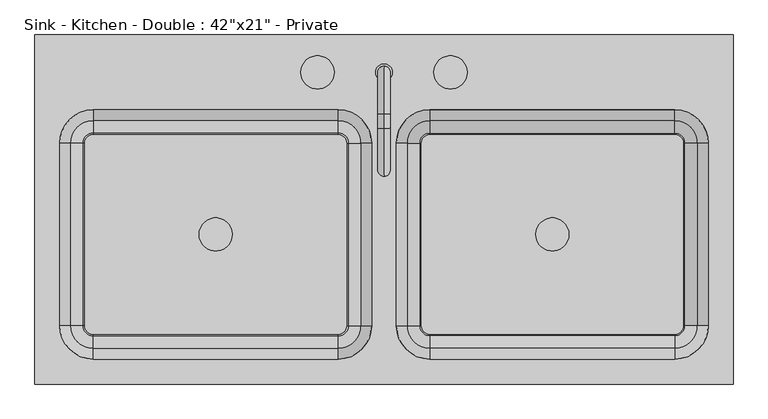
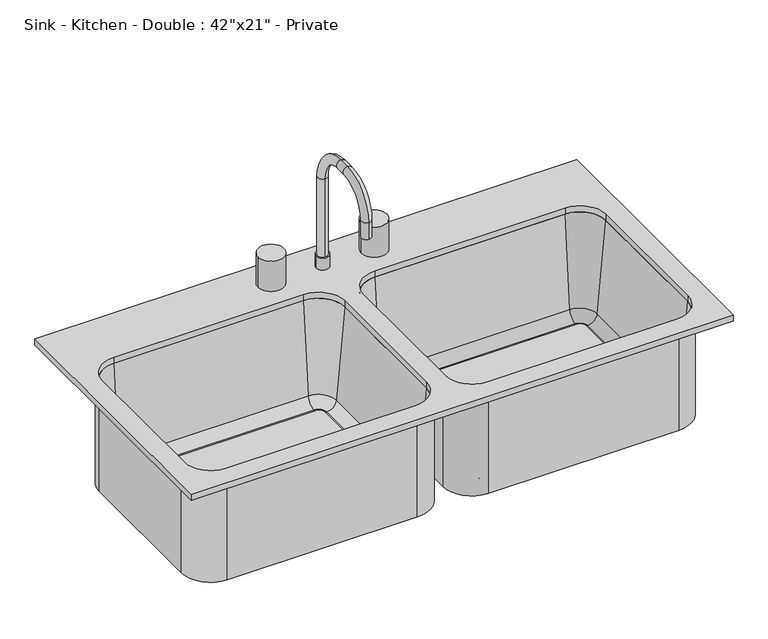
"""IFC4 building model written with IfcOpenShell, lengths in millimetres: flow terminal geometry."""

from ifc_helpers import new_model, si_unit, point, frame, frame_2d, origin, origin_with_axes, place, context, project, spatial, polyline, circle_curve, ellipse_curve, trimmed, segment, composite_curve, outline, extrude, source, transform, mapped, element, save
from ifc_brep_helpers import plane_surface, cylinder_surface, revolved_surface, advanced_brep


def flow_terminal_ad7a5719(model_context):
    return source(origin(), model_context, "Body", "SolidModel", [
        extrude(outline(composite_curve([segment(trimmed(circle_curve(frame_2d((444.5, -165.1)), 12.7), [point((444.5, -152.4))], [point((457.2, -165.1))], False, "CARTESIAN"), True, "CONTINUOUS"), segment(polyline([(457.2, -165.1), (457.2, -444.5)]), True, "CONTINUOUS"), segment(trimmed(circle_curve(frame_2d((444.5, -444.5)), 12.7), [point((457.2, -444.5))], [point((444.5, -457.2))], False, "CARTESIAN"), True, "CONTINUOUS"), segment(polyline([(444.5, -457.2), (69.85, -457.2)]), True, "CONTINUOUS"), segment(trimmed(circle_curve(frame_2d((69.85, -444.5)), 12.7), [point((69.85, -457.2))], [point((57.15, -444.5))], False, "CARTESIAN"), True, "CONTINUOUS"), segment(polyline([(57.15, -444.5), (57.15, -165.1)]), True, "CONTINUOUS"), segment(trimmed(circle_curve(frame_2d((69.85, -165.1)), 12.7), [point((57.15, -165.1))], [point((69.85, -152.4))], False, "CARTESIAN"), True, "CONTINUOUS"), segment(polyline([(69.85, -152.4), (444.5, -152.4)]), True, "CONTINUOUS")], self_intersect=False), holes=[composite_curve([segment(trimmed(circle_curve(frame_2d((257.175, -304.8)), 25.4), [point((231.775, -304.8))], [point((282.575, -304.8))], True, "CARTESIAN"), True, "CONTINUOUS"), segment(trimmed(circle_curve(frame_2d((257.175, -304.8)), 25.4), [point((282.575, -304.8))], [point((231.775, -304.8))], True, "CARTESIAN"), True, "CONTINUOUS")], self_intersect=False)]), frame((0.0, 0.0, -215.9), z_axis=(0.0, 0.0, 1.0), x_axis=(1.0, 0.0, 0.0)), (0.0, 0.0, 1.0), 9.525),
        advanced_brep(
        [(19.05, -165.1, 0.0), (69.85, -114.3, 0.0), (69.85, -107.95, 0.0), (12.7, -165.1, 0.0), (35.5840728, -165.1, -188.9853169), (69.85, -130.8340728, -188.9853169), (54.5615818, -165.1, -206.375), (69.85, -149.8115818, -206.375), (57.15, -165.1, -206.375), (69.85, -152.4, -206.375), (57.15, -165.1, -215.9), (69.85, -152.4, -215.9), (12.7, -165.1, -215.9), (69.85, -107.95, -215.9), (12.7, -444.5, 0.0), (19.05, -444.5, 0.0), (35.5840728, -444.5, -188.9853169), (54.5615818, -444.5, -206.375), (57.15, -444.5, -206.375), (57.15, -444.5, -215.9), (12.7, -444.5, -215.9), (69.85, -495.3, 0.0), (69.85, -501.65, 0.0), (69.85, -478.7659272, -188.9853169), (69.85, -459.7884182, -206.375), (69.85, -457.2, -206.375), (69.85, -457.2, -215.9), (69.85, -501.65, -215.9), (444.5, -501.65, 0.0), (444.5, -495.3, 0.0), (444.5, -478.7659272, -188.9853169), (444.5, -459.7884182, -206.375), (444.5, -457.2, -206.375), (444.5, -457.2, -215.9), (444.5, -501.65, -215.9), (495.3, -444.5, 0.0), (501.65, -444.5, 0.0), (478.7659272, -444.5, -188.9853169), (459.7884182, -444.5, -206.375), (457.2, -444.5, -206.375), (457.2, -444.5, -215.9), (501.65, -444.5, -215.9), (501.65, -165.1, 0.0), (495.3, -165.1, 0.0), (478.7659272, -165.1, -188.9853169), (459.7884182, -165.1, -206.375), (457.2, -165.1, -206.375), (457.2, -165.1, -215.9), (501.65, -165.1, -215.9), (444.5, -114.3, 0.0), (444.5, -107.95, 0.0), (444.5, -130.8340728, -188.9853169), (444.5, -149.8115818, -206.375), (444.5, -152.4, -206.375), (444.5, -152.4, -215.9), (444.5, -107.95, -215.9)],
        [
            (0, 1, circle_curve(frame((69.85, -165.1, 0.0), z_axis=(0.0, 0.0, -1.0), x_axis=(0.0, 1.0, 0.0)), 50.8)),
            (1, 2),
            (2, 3, circle_curve(frame((69.85, -165.1, 0.0), z_axis=(0.0, 0.0, 1.0), x_axis=(0.0, 1.0, 0.0)), 57.15)),
            (3, 0),
            (4, 5, circle_curve(frame((69.85, -165.1, -188.9853169), z_axis=(0.0, 0.0, -1.0), x_axis=(0.0, 1.0, 0.0)), 34.2659272)),
            (5, 1),
            (0, 4),
            (6, 7, circle_curve(frame((69.85, -165.1, -206.375), z_axis=(0.0, 0.0, -1.0), x_axis=(0.0, 1.0, 0.0)), 15.2884182)),
            (7, 5, circle_curve(frame((69.85, -149.8115818, -187.325), z_axis=(1.0, 0.0, 0.0), x_axis=(0.0, -1.0, 0.0)), 19.05)),
            (4, 6, circle_curve(frame((54.5615818, -165.1, -187.325), z_axis=(0.0, -1.0, 0.0), x_axis=(1.0, 0.0, 0.0)), 19.05)),
            (8, 9, circle_curve(frame((69.85, -165.1, -206.375), z_axis=(0.0, 0.0, -1.0), x_axis=(0.0, 1.0, 0.0)), 12.7)),
            (9, 7),
            (6, 8),
            (10, 11, circle_curve(frame((69.85, -165.1, -215.9), z_axis=(0.0, 0.0, -1.0), x_axis=(0.0, 1.0, 0.0)), 12.7)),
            (11, 9),
            (8, 10),
            (12, 13, circle_curve(frame((69.85, -165.1, -215.9), z_axis=(0.0, 0.0, -1.0), x_axis=(0.0, 1.0, 0.0)), 57.15)),
            (13, 11),
            (10, 12),
            (2, 13),
            (12, 3),
            (3, 14),
            (14, 15),
            (15, 0),
            (15, 16),
            (16, 4),
            (16, 17, circle_curve(frame((54.5615818, -444.5, -187.325), z_axis=(0.0, -1.0, 0.0), x_axis=(1.0, 0.0, 0.0)), 19.05)),
            (17, 6),
            (17, 18),
            (18, 8),
            (18, 19),
            (19, 10),
            (19, 20),
            (20, 12),
            (20, 14),
            (21, 15, circle_curve(frame((69.85, -444.5, 0.0), z_axis=(0.0, 0.0, -1.0), x_axis=(-1.0, 0.0, 0.0)), 50.8)),
            (14, 22, circle_curve(frame((69.85, -444.5, 0.0), z_axis=(0.0, 0.0, 1.0), x_axis=(-1.0, 0.0, 0.0)), 57.15)),
            (22, 21),
            (23, 16, circle_curve(frame((69.85, -444.5, -188.9853169), z_axis=(0.0, 0.0, -1.0), x_axis=(-1.0, 0.0, 0.0)), 34.2659272)),
            (21, 23),
            (24, 17, circle_curve(frame((69.85, -444.5, -206.375), z_axis=(0.0, 0.0, -1.0), x_axis=(-1.0, 0.0, 0.0)), 15.2884182)),
            (23, 24, circle_curve(frame((69.85, -459.7884182, -187.325), z_axis=(1.0, 0.0, 0.0), x_axis=(0.0, 1.0, 0.0)), 19.05)),
            (25, 18, circle_curve(frame((69.85, -444.5, -206.375), z_axis=(0.0, 0.0, -1.0), x_axis=(-1.0, 0.0, 0.0)), 12.7)),
            (24, 25),
            (26, 19, circle_curve(frame((69.85, -444.5, -215.9), z_axis=(0.0, 0.0, -1.0), x_axis=(-1.0, 0.0, 0.0)), 12.7)),
            (25, 26),
            (27, 20, circle_curve(frame((69.85, -444.5, -215.9), z_axis=(0.0, 0.0, -1.0), x_axis=(-1.0, 0.0, 0.0)), 57.15)),
            (26, 27),
            (27, 22),
            (22, 28),
            (28, 29),
            (29, 21),
            (29, 30),
            (30, 23),
            (30, 31, circle_curve(frame((444.5, -459.7884182, -187.325), z_axis=(1.0, 0.0, 0.0), x_axis=(0.0, 1.0, 0.0)), 19.05)),
            (31, 24),
            (31, 32),
            (32, 25),
            (32, 33),
            (33, 26),
            (33, 34),
            (34, 27),
            (34, 28),
            (35, 29, circle_curve(frame((444.5, -444.5, 0.0), z_axis=(0.0, 0.0, -1.0), x_axis=(0.0, -1.0, 0.0)), 50.8)),
            (28, 36, circle_curve(frame((444.5, -444.5, 0.0), z_axis=(0.0, 0.0, 1.0), x_axis=(0.0, -1.0, 0.0)), 57.15)),
            (36, 35),
            (37, 30, circle_curve(frame((444.5, -444.5, -188.9853169), z_axis=(0.0, 0.0, -1.0), x_axis=(0.0, -1.0, 0.0)), 34.2659272)),
            (35, 37),
            (38, 31, circle_curve(frame((444.5, -444.5, -206.375), z_axis=(0.0, 0.0, -1.0), x_axis=(0.0, -1.0, 0.0)), 15.2884182)),
            (37, 38, circle_curve(frame((459.7884182, -444.5, -187.325), z_axis=(0.0, 1.0, 0.0), x_axis=(-1.0, 0.0, 0.0)), 19.05)),
            (39, 32, circle_curve(frame((444.5, -444.5, -206.375), z_axis=(0.0, 0.0, -1.0), x_axis=(0.0, -1.0, 0.0)), 12.7)),
            (38, 39),
            (40, 33, circle_curve(frame((444.5, -444.5, -215.9), z_axis=(0.0, 0.0, -1.0), x_axis=(0.0, -1.0, 0.0)), 12.7)),
            (39, 40),
            (41, 34, circle_curve(frame((444.5, -444.5, -215.9), z_axis=(0.0, 0.0, -1.0), x_axis=(0.0, -1.0, 0.0)), 57.15)),
            (40, 41),
            (41, 36),
            (36, 42),
            (42, 43),
            (43, 35),
            (43, 44),
            (44, 37),
            (44, 45, circle_curve(frame((459.7884182, -165.1, -187.325), z_axis=(0.0, 1.0, 0.0), x_axis=(-1.0, 0.0, 0.0)), 19.05)),
            (45, 38),
            (45, 46),
            (46, 39),
            (46, 47),
            (47, 40),
            (47, 48),
            (48, 41),
            (48, 42),
            (49, 43, circle_curve(frame((444.5, -165.1, 0.0), z_axis=(0.0, 0.0, -1.0), x_axis=(1.0, 0.0, 0.0)), 50.8)),
            (42, 50, circle_curve(frame((444.5, -165.1, 0.0), z_axis=(0.0, 0.0, 1.0), x_axis=(1.0, 0.0, 0.0)), 57.15)),
            (50, 49),
            (51, 44, circle_curve(frame((444.5, -165.1, -188.9853169), z_axis=(0.0, 0.0, -1.0), x_axis=(1.0, 0.0, 0.0)), 34.2659272)),
            (49, 51),
            (52, 45, circle_curve(frame((444.5, -165.1, -206.375), z_axis=(0.0, 0.0, -1.0), x_axis=(1.0, 0.0, 0.0)), 15.2884182)),
            (51, 52, circle_curve(frame((444.5, -149.8115818, -187.325), z_axis=(-1.0, 0.0, 0.0), x_axis=(0.0, -1.0, 0.0)), 19.05)),
            (53, 46, circle_curve(frame((444.5, -165.1, -206.375), z_axis=(0.0, 0.0, -1.0), x_axis=(1.0, 0.0, 0.0)), 12.7)),
            (52, 53),
            (54, 47, circle_curve(frame((444.5, -165.1, -215.9), z_axis=(0.0, 0.0, -1.0), x_axis=(1.0, 0.0, 0.0)), 12.7)),
            (53, 54),
            (55, 48, circle_curve(frame((444.5, -165.1, -215.9), z_axis=(0.0, 0.0, -1.0), x_axis=(1.0, 0.0, 0.0)), 57.15)),
            (54, 55),
            (55, 50),
            (50, 2),
            (1, 49),
            (5, 51),
            (7, 52),
            (9, 53),
            (11, 54),
            (13, 55),
        ],
        [
            plane_surface(frame((69.85, -165.1, 0.0), z_axis=(0.0, 0.0, 1.0), x_axis=(0.0, 1.0, 0.0))),
            revolved_surface(polyline([(69.85, -114.3, 0.0), (69.85, -130.8340728, -188.9853169)]), (69.85, -165.1, -914.4), (0.0, 0.0, 1.0)),
            revolved_surface(trimmed(ellipse_curve(frame((69.85, -149.8115818, -187.325), z_axis=(-1.0, 0.0, 0.0), x_axis=(0.0, -1.0, 0.0)), 19.05, 19.05), [point((69.85, -130.8340728, -188.9853169))], [point((69.85, -149.8115818, -206.375))], True, "CARTESIAN"), (69.85, -165.1, -914.4), (0.0, 0.0, 1.0)),
            plane_surface(frame((69.85, -165.1, -206.375), z_axis=(0.0, 0.0, 1.0), x_axis=(0.0, 1.0, 0.0))),
            revolved_surface(polyline([(69.85, -152.4, -206.375), (69.85, -152.4, -215.89999999999998)]), (69.85, -165.1, -914.4), (0.0, 0.0, 1.0)),
            plane_surface(frame((69.85, -165.1, -215.9), z_axis=(0.0, 0.0, -1.0), x_axis=(0.0, 1.0, 0.0))),
            cylinder_surface(frame((69.85, -165.1, -914.4), z_axis=(0.0, 0.0, 1.0), x_axis=(0.0, 1.0, 0.0)), 57.15),
            plane_surface(frame((12.7, -165.1, 0.0), z_axis=(0.0, 0.0, 1.0), x_axis=(0.0, -1.0, 0.0))),
            plane_surface(frame((19.05, -165.1, 0.0), z_axis=(0.9961946980917455, 0.0, 0.0871557427476589), x_axis=(0.0, -1.0, 0.0))),
            revolved_surface(polyline([(73.6115818, -444.5, -187.325), (73.6115818, -165.1, -187.325)]), (54.5615818, -165.1, -187.325), (0.0, -1.0, 0.0)),
            plane_surface(frame((54.5615818, -165.1, -206.375), z_axis=(0.0, 0.0, 1.0), x_axis=(0.0, -1.0, 0.0))),
            plane_surface(frame((57.15, -165.1, -206.375), z_axis=(1.0, 0.0, 0.0), x_axis=(0.0, -1.0, 0.0))),
            plane_surface(frame((57.15, -165.1, -215.9), z_axis=(0.0, 0.0, -1.0), x_axis=(0.0, -1.0, 0.0))),
            plane_surface(frame((12.7, -165.1, -215.9), z_axis=(-1.0, 0.0, 0.0), x_axis=(0.0, -1.0, 0.0))),
            plane_surface(frame((69.85, -444.5, 0.0), z_axis=(0.0, 0.0, 1.0), x_axis=(-1.0, 0.0, 0.0))),
            revolved_surface(polyline([(19.05, -444.5, 0.0), (35.5840728, -444.5, -188.9853169)]), (69.85, -444.5, -914.4), (0.0, 0.0, 1.0)),
            revolved_surface(trimmed(ellipse_curve(frame((54.5615818, -444.5, -187.325), z_axis=(0.0, -1.0, 0.0), x_axis=(1.0, 0.0, 0.0)), 19.05, 19.05), [point((35.5840728, -444.5, -188.9853169))], [point((54.5615818, -444.5, -206.375))], True, "CARTESIAN"), (69.85, -444.5, -914.4), (0.0, 0.0, 1.0)),
            plane_surface(frame((69.85, -444.5, -206.375), z_axis=(0.0, 0.0, 1.0), x_axis=(-1.0, 0.0, 0.0))),
            revolved_surface(polyline([(57.14999999999999, -444.5, -206.375), (57.14999999999999, -444.5, -215.89999999999998)]), (69.85, -444.5, -914.4), (0.0, 0.0, 1.0)),
            plane_surface(frame((69.85, -444.5, -215.9), z_axis=(0.0, 0.0, -1.0), x_axis=(-1.0, 0.0, 0.0))),
            cylinder_surface(frame((69.85, -444.5, -914.4), z_axis=(0.0, 0.0, 1.0), x_axis=(-1.0, 0.0, 0.0)), 57.15),
            plane_surface(frame((69.85, -501.65, 0.0), z_axis=(0.0, 0.0, 1.0), x_axis=(1.0, 0.0, 0.0))),
            plane_surface(frame((69.85, -495.3, 0.0), z_axis=(0.0, 0.9961946980917455, 0.0871557427476589), x_axis=(1.0, 0.0, 0.0))),
            revolved_surface(polyline([(444.5, -440.7384182, -187.325), (69.85, -440.7384182, -187.325)]), (69.85, -459.7884182, -187.325), (1.0, 0.0, 0.0)),
            plane_surface(frame((69.85, -459.7884182, -206.375), z_axis=(0.0, 0.0, 1.0), x_axis=(1.0, 0.0, 0.0))),
            plane_surface(frame((69.85, -457.2, -206.375), z_axis=(0.0, 1.0, 0.0), x_axis=(1.0, 0.0, 0.0))),
            plane_surface(frame((69.85, -457.2, -215.9), z_axis=(0.0, 0.0, -1.0), x_axis=(1.0, 0.0, 0.0))),
            plane_surface(frame((69.85, -501.65, -215.9), z_axis=(0.0, -1.0, 0.0), x_axis=(1.0, 0.0, 0.0))),
            plane_surface(frame((444.5, -444.5, 0.0), z_axis=(0.0, 0.0, 1.0), x_axis=(0.0, -1.0, 0.0))),
            revolved_surface(polyline([(444.5, -495.3, 0.0), (444.5, -478.7659272, -188.9853169)]), (444.5, -444.5, -914.4), (0.0, 0.0, 1.0)),
            revolved_surface(trimmed(ellipse_curve(frame((444.5, -459.7884182, -187.325), z_axis=(1.0, 0.0, 0.0), x_axis=(0.0, 1.0, 0.0)), 19.05, 19.05), [point((444.5, -478.7659272, -188.9853169))], [point((444.5, -459.7884182, -206.375))], True, "CARTESIAN"), (444.5, -444.5, -914.4), (0.0, 0.0, 1.0)),
            plane_surface(frame((444.5, -444.5, -206.375), z_axis=(0.0, 0.0, 1.0), x_axis=(0.0, -1.0, 0.0))),
            revolved_surface(polyline([(444.5, -457.2, -206.375), (444.5, -457.2, -215.89999999999998)]), (444.5, -444.5, -914.4), (0.0, 0.0, 1.0)),
            plane_surface(frame((444.5, -444.5, -215.9), z_axis=(0.0, 0.0, -1.0), x_axis=(0.0, -1.0, 0.0))),
            cylinder_surface(frame((444.5, -444.5, -914.4), z_axis=(0.0, 0.0, 1.0), x_axis=(0.0, -1.0, 0.0)), 57.15),
            plane_surface(frame((501.65, -444.5, 0.0), z_axis=(0.0, 0.0, 1.0), x_axis=(0.0, 1.0, 0.0))),
            plane_surface(frame((495.3, -444.5, 0.0), z_axis=(-0.9961946980917455, 0.0, 0.0871557427476589), x_axis=(0.0, 1.0, 0.0))),
            revolved_surface(polyline([(440.7384182, -165.10000000000002, -187.325), (440.7384182, -444.5, -187.325)]), (459.7884182, -444.5, -187.325), (0.0, 1.0, 0.0)),
            plane_surface(frame((459.7884182, -444.5, -206.375), z_axis=(0.0, 0.0, 1.0), x_axis=(0.0, 1.0, 0.0))),
            plane_surface(frame((457.2, -444.5, -206.375), z_axis=(-1.0, 0.0, 0.0), x_axis=(0.0, 1.0, 0.0))),
            plane_surface(frame((457.2, -444.5, -215.9), z_axis=(0.0, 0.0, -1.0), x_axis=(0.0, 1.0, 0.0))),
            plane_surface(frame((501.65, -444.5, -215.9), z_axis=(1.0, 0.0, 0.0), x_axis=(0.0, 1.0, 0.0))),
            plane_surface(frame((444.5, -165.1, 0.0), z_axis=(0.0, 0.0, 1.0), x_axis=(1.0, 0.0, 0.0))),
            revolved_surface(polyline([(495.3, -165.1, 0.0), (478.7659272, -165.1, -188.9853169)]), (444.5, -165.1, -914.4), (0.0, 0.0, 1.0)),
            revolved_surface(trimmed(ellipse_curve(frame((459.7884182, -165.1, -187.325), z_axis=(0.0, 1.0, 0.0), x_axis=(-1.0, 0.0, 0.0)), 19.05, 19.05), [point((478.7659272, -165.1, -188.9853169))], [point((459.7884182, -165.1, -206.375))], True, "CARTESIAN"), (444.5, -165.1, -914.4), (0.0, 0.0, 1.0)),
            plane_surface(frame((444.5, -165.1, -206.375), z_axis=(0.0, 0.0, 1.0), x_axis=(1.0, 0.0, 0.0))),
            revolved_surface(polyline([(457.2, -165.1, -206.375), (457.2, -165.1, -215.89999999999998)]), (444.5, -165.1, -914.4), (0.0, 0.0, 1.0)),
            plane_surface(frame((444.5, -165.1, -215.9), z_axis=(0.0, 0.0, -1.0), x_axis=(1.0, 0.0, 0.0))),
            cylinder_surface(frame((444.5, -165.1, -914.4), z_axis=(0.0, 0.0, 1.0), x_axis=(1.0, 0.0, 0.0)), 57.15),
            plane_surface(frame((444.5, -107.95, 0.0), z_axis=(0.0, 0.0, 1.0), x_axis=(-1.0, 0.0, 0.0))),
            plane_surface(frame((444.5, -114.3, 0.0), z_axis=(0.0, -0.9961946980917455, 0.0871557427476589), x_axis=(-1.0, 0.0, 0.0))),
            revolved_surface(polyline([(69.85000000000002, -168.8615818, -187.325), (444.5, -168.8615818, -187.325)]), (444.5, -149.8115818, -187.325), (-1.0, 0.0, 0.0)),
            plane_surface(frame((444.5, -149.8115818, -206.375), z_axis=(0.0, 0.0, 1.0), x_axis=(-1.0, 0.0, 0.0))),
            plane_surface(frame((444.5, -152.4, -206.375), z_axis=(0.0, -1.0, 0.0), x_axis=(-1.0, 0.0, 0.0))),
            plane_surface(frame((444.5, -152.4, -215.9), z_axis=(0.0, 0.0, -1.0), x_axis=(-1.0, 0.0, 0.0))),
            plane_surface(frame((444.5, -107.95, -215.9), z_axis=(0.0, 1.0, 0.0), x_axis=(-1.0, 0.0, 0.0))),
        ],
        [
            (0, [[1, 2, 3, 4]]),
            (1, [[5, 6, -1, 7]]),
            (2, [[8, 9, -5, 10]]),
            (3, [[11, 12, -8, 13]]),
            (4, [[14, 15, -11, 16]]),
            (5, [[17, 18, -14, 19]]),
            (6, [[-3, 20, -17, 21]]),
            (7, [[-4, 22, 23, 24]]),
            (8, [[-7, -24, 25, 26]]),
            (9, [[-10, -26, 27, 28]]),
            (10, [[-13, -28, 29, 30]]),
            (11, [[-16, -30, 31, 32]]),
            (12, [[-19, -32, 33, 34]]),
            (13, [[-21, -34, 35, -22]]),
            (14, [[36, -23, 37, 38]]),
            (15, [[39, -25, -36, 40]]),
            (16, [[41, -27, -39, 42]]),
            (17, [[43, -29, -41, 44]]),
            (18, [[45, -31, -43, 46]]),
            (19, [[47, -33, -45, 48]]),
            (20, [[-37, -35, -47, 49]]),
            (21, [[-38, 50, 51, 52]]),
            (22, [[-40, -52, 53, 54]]),
            (23, [[-42, -54, 55, 56]]),
            (24, [[-44, -56, 57, 58]]),
            (25, [[-46, -58, 59, 60]]),
            (26, [[-48, -60, 61, 62]]),
            (27, [[-49, -62, 63, -50]]),
            (28, [[64, -51, 65, 66]]),
            (29, [[67, -53, -64, 68]]),
            (30, [[69, -55, -67, 70]]),
            (31, [[71, -57, -69, 72]]),
            (32, [[73, -59, -71, 74]]),
            (33, [[75, -61, -73, 76]]),
            (34, [[-65, -63, -75, 77]]),
            (35, [[-66, 78, 79, 80]]),
            (36, [[-68, -80, 81, 82]]),
            (37, [[-70, -82, 83, 84]]),
            (38, [[-72, -84, 85, 86]]),
            (39, [[-74, -86, 87, 88]]),
            (40, [[-76, -88, 89, 90]]),
            (41, [[-77, -90, 91, -78]]),
            (42, [[92, -79, 93, 94]]),
            (43, [[95, -81, -92, 96]]),
            (44, [[97, -83, -95, 98]]),
            (45, [[99, -85, -97, 100]]),
            (46, [[101, -87, -99, 102]]),
            (47, [[103, -89, -101, 104]]),
            (48, [[-93, -91, -103, 105]]),
            (49, [[-94, 106, -2, 107]]),
            (50, [[-96, -107, -6, 108]]),
            (51, [[-98, -108, -9, 109]]),
            (52, [[-100, -109, -12, 110]]),
            (53, [[-102, -110, -15, 111]]),
            (54, [[-104, -111, -18, 112]]),
            (55, [[-105, -112, -20, -106]]),
        ],
    ),
        extrude(outline(composite_curve([segment(trimmed(circle_curve(frame_2d((-69.85, -165.1)), 12.7), [point((-69.85, -152.4))], [point((-57.15, -165.1))], False, "CARTESIAN"), True, "CONTINUOUS"), segment(polyline([(-57.15, -165.1), (-57.15, -444.5)]), True, "CONTINUOUS"), segment(trimmed(circle_curve(frame_2d((-69.85, -444.5)), 12.7), [point((-57.15, -444.5))], [point((-69.85, -457.2))], False, "CARTESIAN"), True, "CONTINUOUS"), segment(polyline([(-69.85, -457.2), (-444.5, -457.2)]), True, "CONTINUOUS"), segment(trimmed(circle_curve(frame_2d((-444.5, -444.5)), 12.7), [point((-444.5, -457.2))], [point((-457.2, -444.5))], False, "CARTESIAN"), True, "CONTINUOUS"), segment(polyline([(-457.2, -444.5), (-457.2, -165.1)]), True, "CONTINUOUS"), segment(trimmed(circle_curve(frame_2d((-444.5, -165.1)), 12.7), [point((-457.2, -165.1))], [point((-444.5, -152.4))], False, "CARTESIAN"), True, "CONTINUOUS"), segment(polyline([(-444.5, -152.4), (-69.85, -152.4)]), True, "CONTINUOUS")], self_intersect=False), holes=[composite_curve([segment(trimmed(circle_curve(frame_2d((-257.175, -304.8)), 25.4), [point((-282.575, -304.8))], [point((-231.775, -304.8))], True, "CARTESIAN"), True, "CONTINUOUS"), segment(trimmed(circle_curve(frame_2d((-257.175, -304.8)), 25.4), [point((-231.775, -304.8))], [point((-282.575, -304.8))], True, "CARTESIAN"), True, "CONTINUOUS")], self_intersect=False)]), frame((0.0, 0.0, -215.9), z_axis=(0.0, 0.0, 1.0), x_axis=(1.0, 0.0, 0.0)), (0.0, 0.0, 1.0), 9.525),
        advanced_brep(
        [(-12.7, -165.1, -215.9), (-69.85, -107.95, -215.9), (-69.85, -107.95, 0.0), (-12.7, -165.1, 0.0), (-57.15, -165.1, -215.9), (-69.85, -152.4, -215.9), (-57.15, -165.1, -206.375), (-69.85, -152.4, -206.375), (-54.5615818, -165.1, -206.375), (-69.85, -149.8115818, -206.375), (-35.5840728, -165.1, -188.9853169), (-69.85, -130.8340728, -188.9853169), (-19.05, -165.1, 0.0), (-69.85, -114.3, 0.0), (-12.7, -444.5, 0.0), (-12.7, -444.5, -215.9), (-57.15, -444.5, -215.9), (-57.15, -444.5, -206.375), (-54.5615818, -444.5, -206.375), (-35.5840728, -444.5, -188.9853169), (-19.05, -444.5, 0.0), (-69.85, -501.65, -215.9), (-69.85, -501.65, 0.0), (-69.85, -457.2, -215.9), (-69.85, -457.2, -206.375), (-69.85, -459.7884182, -206.375), (-69.85, -478.7659272, -188.9853169), (-69.85, -495.3, 0.0), (-444.5, -501.65, 0.0), (-444.5, -501.65, -215.9), (-444.5, -457.2, -215.9), (-444.5, -457.2, -206.375), (-444.5, -459.7884182, -206.375), (-444.5, -478.7659272, -188.9853169), (-444.5, -495.3, 0.0), (-501.65, -444.5, -215.9), (-501.65, -444.5, 0.0), (-457.2, -444.5, -215.9), (-457.2, -444.5, -206.375), (-459.7884182, -444.5, -206.375), (-478.7659272, -444.5, -188.9853169), (-495.3, -444.5, 0.0), (-501.65, -165.1, 0.0), (-501.65, -165.1, -215.9), (-457.2, -165.1, -215.9), (-457.2, -165.1, -206.375), (-459.7884182, -165.1, -206.375), (-478.7659272, -165.1, -188.9853169), (-495.3, -165.1, 0.0), (-444.5, -107.95, -215.9), (-444.5, -107.95, 0.0), (-444.5, -152.4, -215.9), (-444.5, -152.4, -206.375), (-444.5, -149.8115818, -206.375), (-444.5, -130.8340728, -188.9853169), (-444.5, -114.3, 0.0)],
        [
            (0, 1, circle_curve(frame((-69.85, -165.1, -215.9), z_axis=(0.0, 0.0, 1.0), x_axis=(0.0, 1.0, 0.0)), 57.15)),
            (1, 2),
            (2, 3, circle_curve(frame((-69.85, -165.1, 0.0), z_axis=(0.0, 0.0, -1.0), x_axis=(0.0, 1.0, 0.0)), 57.15)),
            (3, 0),
            (4, 5, circle_curve(frame((-69.85, -165.1, -215.9), z_axis=(0.0, 0.0, 1.0), x_axis=(0.0, 1.0, 0.0)), 12.7)),
            (5, 1),
            (0, 4),
            (6, 7, circle_curve(frame((-69.85, -165.1, -206.375), z_axis=(0.0, 0.0, 1.0), x_axis=(0.0, 1.0, 0.0)), 12.7)),
            (7, 5),
            (4, 6),
            (8, 9, circle_curve(frame((-69.85, -165.1, -206.375), z_axis=(0.0, 0.0, 1.0), x_axis=(0.0, 1.0, 0.0)), 15.2884182)),
            (9, 7),
            (6, 8),
            (10, 11, circle_curve(frame((-69.85, -165.1, -188.9853169), z_axis=(0.0, 0.0, 1.0), x_axis=(0.0, 1.0, 0.0)), 34.2659272)),
            (11, 9, circle_curve(frame((-69.85, -149.8115818, -187.325), z_axis=(-1.0, 0.0, 0.0), x_axis=(0.0, 1.0, 0.0)), 19.05)),
            (8, 10, circle_curve(frame((-54.5615818, -165.1, -187.325), z_axis=(-1.3096190798478347e-12, -1.0, 0.0), x_axis=(1.0, -1.3096190798478347e-12, 0.0)), 19.05)),
            (12, 13, circle_curve(frame((-69.85, -165.1, 0.0), z_axis=(0.0, 0.0, 1.0), x_axis=(0.0, 1.0, 0.0)), 50.8)),
            (13, 11),
            (10, 12),
            (2, 13),
            (12, 3),
            (3, 14),
            (14, 15),
            (15, 0),
            (15, 16),
            (16, 4),
            (16, 17),
            (17, 6),
            (17, 18),
            (18, 8),
            (18, 19, circle_curve(frame((-54.5615818, -444.5, -187.325), z_axis=(0.0, -1.0, 0.0), x_axis=(1.0, 0.0, 0.0)), 19.05)),
            (19, 10),
            (19, 20),
            (20, 12),
            (20, 14),
            (21, 15, circle_curve(frame((-69.85, -444.5, -215.9), z_axis=(0.0, 0.0, 1.0), x_axis=(1.0, 0.0, 0.0)), 57.15)),
            (14, 22, circle_curve(frame((-69.85, -444.5, 0.0), z_axis=(0.0, 0.0, -1.0), x_axis=(1.0, 0.0, 0.0)), 57.15)),
            (22, 21),
            (23, 16, circle_curve(frame((-69.85, -444.5, -215.9), z_axis=(0.0, 0.0, 1.0), x_axis=(1.0, 0.0, 0.0)), 12.7)),
            (21, 23),
            (24, 17, circle_curve(frame((-69.85, -444.5, -206.375), z_axis=(0.0, 0.0, 1.0), x_axis=(1.0, 0.0, 0.0)), 12.7)),
            (23, 24),
            (25, 18, circle_curve(frame((-69.85, -444.5, -206.375), z_axis=(0.0, 0.0, 1.0), x_axis=(1.0, 0.0, 0.0)), 15.2884182)),
            (24, 25),
            (26, 19, circle_curve(frame((-69.85, -444.5, -188.9853169), z_axis=(0.0, 0.0, 1.0), x_axis=(1.0, 0.0, 0.0)), 34.2659272)),
            (25, 26, circle_curve(frame((-69.85, -459.7884182, -187.325), z_axis=(-1.0, 0.0, 0.0), x_axis=(0.0, -1.0, 0.0)), 19.05)),
            (27, 20, circle_curve(frame((-69.85, -444.5, 0.0), z_axis=(0.0, 0.0, 1.0), x_axis=(1.0, 0.0, 0.0)), 50.8)),
            (26, 27),
            (27, 22),
            (22, 28),
            (28, 29),
            (29, 21),
            (29, 30),
            (30, 23),
            (30, 31),
            (31, 24),
            (31, 32),
            (32, 25),
            (32, 33, circle_curve(frame((-444.5, -459.7884182, -187.325), z_axis=(-1.0, 0.0, 0.0), x_axis=(0.0, -1.0, 0.0)), 19.05)),
            (33, 26),
            (33, 34),
            (34, 27),
            (34, 28),
            (35, 29, circle_curve(frame((-444.5, -444.5, -215.9), z_axis=(0.0, 0.0, 1.0), x_axis=(0.0, -1.0, 0.0)), 57.15)),
            (28, 36, circle_curve(frame((-444.5, -444.5, 0.0), z_axis=(0.0, 0.0, -1.0), x_axis=(0.0, -1.0, 0.0)), 57.15)),
            (36, 35),
            (37, 30, circle_curve(frame((-444.5, -444.5, -215.9), z_axis=(0.0, 0.0, 1.0), x_axis=(0.0, -1.0, 0.0)), 12.7)),
            (35, 37),
            (38, 31, circle_curve(frame((-444.5, -444.5, -206.375), z_axis=(0.0, 0.0, 1.0), x_axis=(0.0, -1.0, 0.0)), 12.7)),
            (37, 38),
            (39, 32, circle_curve(frame((-444.5, -444.5, -206.375), z_axis=(0.0, 0.0, 1.0), x_axis=(0.0, -1.0, 0.0)), 15.2884182)),
            (38, 39),
            (40, 33, circle_curve(frame((-444.5, -444.5, -188.9853169), z_axis=(0.0, 0.0, 1.0), x_axis=(0.0, -1.0, 0.0)), 34.2659272)),
            (39, 40, circle_curve(frame((-459.7884182, -444.5, -187.325), z_axis=(0.0, 1.0, 0.0), x_axis=(-1.0, 0.0, 0.0)), 19.05)),
            (41, 34, circle_curve(frame((-444.5, -444.5, 0.0), z_axis=(0.0, 0.0, 1.0), x_axis=(0.0, -1.0, 0.0)), 50.8)),
            (40, 41),
            (41, 36),
            (36, 42),
            (42, 43),
            (43, 35),
            (43, 44),
            (44, 37),
            (44, 45),
            (45, 38),
            (45, 46),
            (46, 39),
            (46, 47, circle_curve(frame((-459.7884182, -165.1, -187.325), z_axis=(0.0, 1.0, 0.0), x_axis=(-1.0, 0.0, 0.0)), 19.05)),
            (47, 40),
            (47, 48),
            (48, 41),
            (48, 42),
            (49, 43, circle_curve(frame((-444.5, -165.1, -215.9), z_axis=(0.0, 0.0, 1.0), x_axis=(-1.0, 0.0, 0.0)), 57.15)),
            (42, 50, circle_curve(frame((-444.5, -165.1, 0.0), z_axis=(0.0, 0.0, -1.0), x_axis=(-1.0, 0.0, 0.0)), 57.15)),
            (50, 49),
            (51, 44, circle_curve(frame((-444.5, -165.1, -215.9), z_axis=(0.0, 0.0, 1.0), x_axis=(-1.0, 0.0, 0.0)), 12.7)),
            (49, 51),
            (52, 45, circle_curve(frame((-444.5, -165.1, -206.375), z_axis=(0.0, 0.0, 1.0), x_axis=(-1.0, 0.0, 0.0)), 12.7)),
            (51, 52),
            (53, 46, circle_curve(frame((-444.5, -165.1, -206.375), z_axis=(0.0, 0.0, 1.0), x_axis=(-1.0, 0.0, 0.0)), 15.2884182)),
            (52, 53),
            (54, 47, circle_curve(frame((-444.5, -165.1, -188.9853169), z_axis=(0.0, 0.0, 1.0), x_axis=(-1.0, 0.0, 0.0)), 34.2659272)),
            (53, 54, circle_curve(frame((-444.5, -149.8115818, -187.325), z_axis=(1.0, 0.0, 0.0), x_axis=(0.0, 1.0, 0.0)), 19.05)),
            (55, 48, circle_curve(frame((-444.5, -165.1, 0.0), z_axis=(0.0, 0.0, 1.0), x_axis=(-1.0, 0.0, 0.0)), 50.8)),
            (54, 55),
            (55, 50),
            (50, 2),
            (1, 49),
            (5, 51),
            (7, 52),
            (9, 53),
            (11, 54),
            (13, 55),
        ],
        [
            cylinder_surface(frame((-69.85, -165.1, -914.4), z_axis=(0.0, 0.0, -1.0), x_axis=(0.0, 1.0, 0.0)), 57.15),
            plane_surface(frame((-69.85, -165.1, -215.9), z_axis=(0.0, 0.0, -1.0), x_axis=(0.0, 1.0, 0.0))),
            revolved_surface(polyline([(-69.85, -152.4, -215.89999999999998), (-69.85, -152.4, -206.375)]), (-69.85, -165.1, -914.4), (0.0, 0.0, -1.0)),
            plane_surface(frame((-69.85, -165.1, -206.375), z_axis=(0.0, 0.0, 1.0), x_axis=(0.0, 1.0, 0.0))),
            revolved_surface(trimmed(ellipse_curve(frame((-69.85, -149.8115818, -187.325), z_axis=(1.0, 0.0, 0.0), x_axis=(0.0, 1.0, 0.0)), 19.05, 19.05), [point((-69.85, -149.8115818, -206.375))], [point((-69.85, -130.8340728, -188.9853169))], True, "CARTESIAN"), (-69.85, -165.1, -914.4), (0.0, 0.0, -1.0)),
            revolved_surface(polyline([(-69.85, -130.8340728, -188.9853169), (-69.85, -114.3, 0.0)]), (-69.85, -165.1, -914.4), (0.0, 0.0, -1.0)),
            plane_surface(frame((-69.85, -165.1, 0.0), z_axis=(0.0, 0.0, 1.0), x_axis=(0.0, 1.0, 0.0))),
            plane_surface(frame((-12.7, -165.1, 0.0), z_axis=(1.0, 0.0, 0.0), x_axis=(0.0, -1.0, 0.0))),
            plane_surface(frame((-12.7, -165.1, -215.9), z_axis=(0.0, 0.0, -1.0), x_axis=(0.0, -1.0, 0.0))),
            plane_surface(frame((-57.15, -165.1, -215.9), z_axis=(-1.0, 0.0, 0.0), x_axis=(0.0, -1.0, 0.0))),
            plane_surface(frame((-57.15, -165.1, -206.375), z_axis=(0.0, 0.0, 1.0), x_axis=(0.0, -1.0, 0.0))),
            revolved_surface(polyline([(-35.5115818, -444.5, -187.325), (-35.5115818, -165.09999999997504, -187.325)]), (-54.5615818, -165.1, -187.325), (0.0, -1.0, 0.0)),
            plane_surface(frame((-35.5840728, -165.1, -188.9853169), z_axis=(-0.9961946980917444, 0.0, 0.08715574274767054), x_axis=(0.0, -1.0, 0.0))),
            plane_surface(frame((-19.05, -165.1, 0.0), z_axis=(0.0, 0.0, 1.0), x_axis=(0.0, -1.0, 0.0))),
            cylinder_surface(frame((-69.85, -444.5, -914.4), z_axis=(0.0, 0.0, -1.0), x_axis=(1.0, 0.0, 0.0)), 57.15),
            plane_surface(frame((-69.85, -444.5, -215.9), z_axis=(0.0, 0.0, -1.0), x_axis=(1.0, 0.0, 0.0))),
            revolved_surface(polyline([(-57.14999999999999, -444.5, -215.89999999999998), (-57.14999999999999, -444.5, -206.375)]), (-69.85, -444.5, -914.4), (0.0, 0.0, -1.0)),
            plane_surface(frame((-69.85, -444.5, -206.375), z_axis=(0.0, 0.0, 1.0), x_axis=(1.0, 0.0, 0.0))),
            revolved_surface(trimmed(ellipse_curve(frame((-54.5615818, -444.5, -187.325), z_axis=(0.0, -1.0, 0.0), x_axis=(1.0, 0.0, 0.0)), 19.05, 19.05), [point((-54.5615818, -444.5, -206.375))], [point((-35.5840728, -444.5, -188.9853169))], True, "CARTESIAN"), (-69.85, -444.5, -914.4), (0.0, 0.0, -1.0)),
            revolved_surface(polyline([(-35.5840728, -444.5, -188.9853169), (-19.05, -444.5, 0.0)]), (-69.85, -444.5, -914.4), (0.0, 0.0, -1.0)),
            plane_surface(frame((-69.85, -444.5, 0.0), z_axis=(0.0, 0.0, 1.0), x_axis=(1.0, 0.0, 0.0))),
            plane_surface(frame((-69.85, -501.65, 0.0), z_axis=(0.0, -1.0, 0.0), x_axis=(-1.0, 0.0, 0.0))),
            plane_surface(frame((-69.85, -501.65, -215.9), z_axis=(0.0, 0.0, -1.0), x_axis=(-1.0, 0.0, 0.0))),
            plane_surface(frame((-69.85, -457.2, -215.9), z_axis=(0.0, 1.0, 0.0), x_axis=(-1.0, 0.0, 0.0))),
            plane_surface(frame((-69.85, -457.2, -206.375), z_axis=(0.0, 0.0, 1.0), x_axis=(-1.0, 0.0, 0.0))),
            revolved_surface(polyline([(-444.5, -478.83841820000004, -187.325), (-69.85, -478.83841820000004, -187.325)]), (-69.85, -459.7884182, -187.325), (-1.0, 0.0, 0.0)),
            plane_surface(frame((-69.85, -478.7659272, -188.9853169), z_axis=(0.0, 0.9961946980917444, 0.08715574274767054), x_axis=(-1.0, 0.0, 0.0))),
            plane_surface(frame((-69.85, -495.3, 0.0), z_axis=(0.0, 0.0, 1.0), x_axis=(-1.0, 0.0, 0.0))),
            cylinder_surface(frame((-444.5, -444.5, -914.4), z_axis=(0.0, 0.0, -1.0), x_axis=(0.0, -1.0, 0.0)), 57.15),
            plane_surface(frame((-444.5, -444.5, -215.9), z_axis=(0.0, 0.0, -1.0), x_axis=(0.0, -1.0, 0.0))),
            revolved_surface(polyline([(-444.5, -457.2, -215.89999999999998), (-444.5, -457.2, -206.375)]), (-444.5, -444.5, -914.4), (0.0, 0.0, -1.0)),
            plane_surface(frame((-444.5, -444.5, -206.375), z_axis=(0.0, 0.0, 1.0), x_axis=(0.0, -1.0, 0.0))),
            revolved_surface(trimmed(ellipse_curve(frame((-444.5, -459.7884182, -187.325), z_axis=(-1.0, 0.0, 0.0), x_axis=(0.0, -1.0, 0.0)), 19.05, 19.05), [point((-444.5, -459.7884182, -206.375))], [point((-444.5, -478.7659272, -188.9853169))], True, "CARTESIAN"), (-444.5, -444.5, -914.4), (0.0, 0.0, -1.0)),
            revolved_surface(polyline([(-444.5, -478.7659272, -188.9853169), (-444.5, -495.3, 0.0)]), (-444.5, -444.5, -914.4), (0.0, 0.0, -1.0)),
            plane_surface(frame((-444.5, -444.5, 0.0), z_axis=(0.0, 0.0, 1.0), x_axis=(0.0, -1.0, 0.0))),
            plane_surface(frame((-501.65, -444.5, 0.0), z_axis=(-1.0, 0.0, 0.0), x_axis=(0.0, 1.0, 0.0))),
            plane_surface(frame((-501.65, -444.5, -215.9), z_axis=(0.0, 0.0, -1.0), x_axis=(0.0, 1.0, 0.0))),
            plane_surface(frame((-457.2, -444.5, -215.9), z_axis=(1.0, 0.0, 0.0), x_axis=(0.0, 1.0, 0.0))),
            plane_surface(frame((-457.2, -444.5, -206.375), z_axis=(0.0, 0.0, 1.0), x_axis=(0.0, 1.0, 0.0))),
            revolved_surface(polyline([(-478.83841820000004, -165.10000000000002, -187.325), (-478.83841820000004, -444.5, -187.325)]), (-459.7884182, -444.5, -187.325), (0.0, 1.0, 0.0)),
            plane_surface(frame((-478.7659272, -444.5, -188.9853169), z_axis=(0.9961946980917444, 0.0, 0.08715574274767054), x_axis=(0.0, 1.0, 0.0))),
            plane_surface(frame((-495.3, -444.5, 0.0), z_axis=(0.0, 0.0, 1.0), x_axis=(0.0, 1.0, 0.0))),
            cylinder_surface(frame((-444.5, -165.1, -914.4), z_axis=(0.0, 0.0, -1.0), x_axis=(-1.0, 0.0, 0.0)), 57.15),
            plane_surface(frame((-444.5, -165.1, -215.9), z_axis=(0.0, 0.0, -1.0), x_axis=(-1.0, 0.0, 0.0))),
            revolved_surface(polyline([(-457.2, -165.1, -215.89999999999998), (-457.2, -165.1, -206.375)]), (-444.5, -165.1, -914.4), (0.0, 0.0, -1.0)),
            plane_surface(frame((-444.5, -165.1, -206.375), z_axis=(0.0, 0.0, 1.0), x_axis=(-1.0, 0.0, 0.0))),
            revolved_surface(trimmed(ellipse_curve(frame((-459.7884182, -165.1, -187.325), z_axis=(0.0, 1.0, 0.0), x_axis=(-1.0, 0.0, 0.0)), 19.05, 19.05), [point((-459.7884182, -165.1, -206.375))], [point((-478.7659272, -165.1, -188.9853169))], True, "CARTESIAN"), (-444.5, -165.1, -914.4), (0.0, 0.0, -1.0)),
            revolved_surface(polyline([(-478.7659272, -165.1, -188.9853169), (-495.3, -165.1, 0.0)]), (-444.5, -165.1, -914.4), (0.0, 0.0, -1.0)),
            plane_surface(frame((-444.5, -165.1, 0.0), z_axis=(0.0, 0.0, 1.0), x_axis=(-1.0, 0.0, 0.0))),
            plane_surface(frame((-444.5, -107.95, 0.0), z_axis=(0.0, 1.0, 0.0), x_axis=(1.0, 0.0, 0.0))),
            plane_surface(frame((-444.5, -107.95, -215.9), z_axis=(0.0, 0.0, -1.0), x_axis=(1.0, 0.0, 0.0))),
            plane_surface(frame((-444.5, -152.4, -215.9), z_axis=(0.0, -1.0, 0.0), x_axis=(1.0, 0.0, 0.0))),
            plane_surface(frame((-444.5, -152.4, -206.375), z_axis=(0.0, 0.0, 1.0), x_axis=(1.0, 0.0, 0.0))),
            revolved_surface(polyline([(-69.85000000000002, -130.7615818, -187.325), (-444.5, -130.7615818, -187.325)]), (-444.5, -149.8115818, -187.325), (1.0, 0.0, 0.0)),
            plane_surface(frame((-444.5, -130.8340728, -188.9853169), z_axis=(0.0, -0.9961946980917444, 0.08715574274767054), x_axis=(1.0, 0.0, 0.0))),
            plane_surface(frame((-444.5, -114.3, 0.0), z_axis=(0.0, 0.0, 1.0), x_axis=(1.0, 0.0, 0.0))),
        ],
        [
            (0, [[1, 2, 3, 4]]),
            (1, [[5, 6, -1, 7]]),
            (2, [[8, 9, -5, 10]]),
            (3, [[11, 12, -8, 13]]),
            (4, [[14, 15, -11, 16]]),
            (5, [[17, 18, -14, 19]]),
            (6, [[-3, 20, -17, 21]]),
            (7, [[-4, 22, 23, 24]]),
            (8, [[-7, -24, 25, 26]]),
            (9, [[-10, -26, 27, 28]]),
            (10, [[-13, -28, 29, 30]]),
            (11, [[-16, -30, 31, 32]]),
            (12, [[-19, -32, 33, 34]]),
            (13, [[-21, -34, 35, -22]]),
            (14, [[36, -23, 37, 38]]),
            (15, [[39, -25, -36, 40]]),
            (16, [[41, -27, -39, 42]]),
            (17, [[43, -29, -41, 44]]),
            (18, [[45, -31, -43, 46]]),
            (19, [[47, -33, -45, 48]]),
            (20, [[-37, -35, -47, 49]]),
            (21, [[-38, 50, 51, 52]]),
            (22, [[-40, -52, 53, 54]]),
            (23, [[-42, -54, 55, 56]]),
            (24, [[-44, -56, 57, 58]]),
            (25, [[-46, -58, 59, 60]]),
            (26, [[-48, -60, 61, 62]]),
            (27, [[-49, -62, 63, -50]]),
            (28, [[64, -51, 65, 66]]),
            (29, [[67, -53, -64, 68]]),
            (30, [[69, -55, -67, 70]]),
            (31, [[71, -57, -69, 72]]),
            (32, [[73, -59, -71, 74]]),
            (33, [[75, -61, -73, 76]]),
            (34, [[-65, -63, -75, 77]]),
            (35, [[-66, 78, 79, 80]]),
            (36, [[-68, -80, 81, 82]]),
            (37, [[-70, -82, 83, 84]]),
            (38, [[-72, -84, 85, 86]]),
            (39, [[-74, -86, 87, 88]]),
            (40, [[-76, -88, 89, 90]]),
            (41, [[-77, -90, 91, -78]]),
            (42, [[92, -79, 93, 94]]),
            (43, [[95, -81, -92, 96]]),
            (44, [[97, -83, -95, 98]]),
            (45, [[99, -85, -97, 100]]),
            (46, [[101, -87, -99, 102]]),
            (47, [[103, -89, -101, 104]]),
            (48, [[-93, -91, -103, 105]]),
            (49, [[-94, 106, -2, 107]]),
            (50, [[-96, -107, -6, 108]]),
            (51, [[-98, -108, -9, 109]]),
            (52, [[-100, -109, -12, 110]]),
            (53, [[-102, -110, -15, 111]]),
            (54, [[-104, -111, -18, 112]]),
            (55, [[-105, -112, -20, -106]]),
        ],
    ),
        extrude(outline(polyline([(533.4, 0.0), (533.4, -533.4), (-533.4, -533.4), (-533.4, 0.0), (533.4, 0.0)]), holes=[composite_curve([segment(polyline([(-69.85, -114.3), (-444.5, -114.3)]), True, "CONTINUOUS"), segment(trimmed(circle_curve(frame_2d((-444.5, -165.1)), 50.8), [point((-444.5, -114.3))], [point((-495.3, -165.1))], True, "CARTESIAN"), True, "CONTINUOUS"), segment(polyline([(-495.3, -165.1), (-495.3, -444.5)]), True, "CONTINUOUS"), segment(trimmed(circle_curve(frame_2d((-444.5, -444.5)), 50.8), [point((-495.3, -444.5))], [point((-444.5, -495.3))], True, "CARTESIAN"), True, "CONTINUOUS"), segment(polyline([(-444.5, -495.3), (-69.85, -495.3)]), True, "CONTINUOUS"), segment(trimmed(circle_curve(frame_2d((-69.85, -444.5)), 50.8), [point((-69.85, -495.3))], [point((-19.05, -444.5))], True, "CARTESIAN"), True, "CONTINUOUS"), segment(polyline([(-19.05, -444.5), (-19.05, -165.1)]), True, "CONTINUOUS"), segment(trimmed(circle_curve(frame_2d((-69.85, -165.1)), 50.8), [point((-19.05, -165.1))], [point((-69.85, -114.3))], True, "CARTESIAN"), True, "CONTINUOUS")], self_intersect=False), composite_curve([segment(polyline([(69.85, -495.3), (444.5, -495.3)]), True, "CONTINUOUS"), segment(trimmed(circle_curve(frame_2d((444.5, -444.5)), 50.8), [point((444.5, -495.3))], [point((495.3, -444.5))], True, "CARTESIAN"), True, "CONTINUOUS"), segment(polyline([(495.3, -444.5), (495.3, -165.1)]), True, "CONTINUOUS"), segment(trimmed(circle_curve(frame_2d((444.5, -165.1)), 50.8), [point((495.3, -165.1))], [point((444.5, -114.3))], True, "CARTESIAN"), True, "CONTINUOUS"), segment(polyline([(444.5, -114.3), (69.85, -114.3)]), True, "CONTINUOUS"), segment(trimmed(circle_curve(frame_2d((69.85, -165.1)), 50.8), [point((69.85, -114.3))], [point((19.05, -165.1))], True, "CARTESIAN"), True, "CONTINUOUS"), segment(polyline([(19.05, -165.1), (19.05, -444.5)]), True, "CONTINUOUS"), segment(trimmed(circle_curve(frame_2d((69.85, -444.5)), 50.8), [point((19.05, -444.5))], [point((69.85, -495.3))], True, "CARTESIAN"), True, "CONTINUOUS")], self_intersect=False)]), origin_with_axes(), (0.0, 0.0, 1.0), 12.7),
        extrude(outline(composite_curve([segment(trimmed(circle_curve(frame_2d((-257.175, -304.8)), 25.4), [point((-282.575, -304.8))], [point((-231.775, -304.8))], False, "CARTESIAN"), True, "CONTINUOUS"), segment(trimmed(circle_curve(frame_2d((-257.175, -304.8)), 25.4), [point((-231.775, -304.8))], [point((-282.575, -304.8))], False, "CARTESIAN"), True, "CONTINUOUS")], self_intersect=False)), frame((0.0, 0.0, -215.9), z_axis=(0.0, 0.0, 1.0), x_axis=(1.0, 0.0, 0.0)), (0.0, 0.0, 1.0), 9.525),
        extrude(outline(composite_curve([segment(trimmed(circle_curve(frame_2d((257.175, -304.8)), 25.4), [point((231.775, -304.8))], [point((282.575, -304.8))], False, "CARTESIAN"), True, "CONTINUOUS"), segment(trimmed(circle_curve(frame_2d((257.175, -304.8)), 25.4), [point((282.575, -304.8))], [point((231.775, -304.8))], False, "CARTESIAN"), True, "CONTINUOUS")], self_intersect=False)), frame((0.0, 0.0, -215.9), z_axis=(0.0, 0.0, 1.0), x_axis=(1.0, 0.0, 0.0)), (0.0, 0.0, 1.0), 9.525),
        advanced_brep(
        [(-12.7, -57.15, 12.7), (12.7, -57.15, 12.7), (0.0, -47.625, 200.025), (0.0, -66.675, 200.025), (0.0, -66.675, 38.1), (0.0, -47.625, 38.1), (0.0, -120.65, 273.05), (0.0, -120.65, 254.0), (0.0, -142.875, 273.05), (0.0, -142.875, 254.0), (0.0, -215.9, 200.025), (0.0, -196.85, 200.025), (0.0, -215.9, 165.1), (0.0, -196.85, 165.1), (-12.7, -57.15, 38.1), (12.7, -57.15, 38.1)],
        [
            (0, 1, circle_curve(frame((0.0, -57.15, 12.7), z_axis=(0.0, 0.0, -1.0), x_axis=(1.0, 0.0, 0.0)), 12.7)),
            (1, 0, circle_curve(frame((0.0, -57.15, 12.7), z_axis=(0.0, 0.0, -1.0), x_axis=(1.0, 0.0, 0.0)), 12.7)),
            (2, 3, circle_curve(frame((0.0, -57.15, 200.025), z_axis=(0.0, 0.0, -1.0), x_axis=(0.0, -1.0, 0.0)), 9.525)),
            (3, 4),
            (4, 5, circle_curve(frame((0.0, -57.15, 38.1), z_axis=(0.0, 0.0, 1.0), x_axis=(0.0, -1.0, 0.0)), 9.525)),
            (5, 2),
            (3, 2, circle_curve(frame((0.0, -57.15, 200.025), z_axis=(0.0, 0.0, -1.0), x_axis=(0.0, -1.0, 0.0)), 9.525)),
            (5, 4, circle_curve(frame((0.0, -57.15, 38.1), z_axis=(0.0, 0.0, 1.0), x_axis=(0.0, -1.0, 0.0)), 9.525)),
            (2, 6, circle_curve(frame((0.0, -120.65, 200.025), z_axis=(1.0, 0.0, 0.0), x_axis=(0.0, 1.0, 0.0)), 73.025)),
            (6, 7, circle_curve(frame((0.0, -120.65, 263.525), z_axis=(0.0, 1.0, 0.0), x_axis=(0.0, 0.0, -1.0)), 9.525)),
            (7, 3, circle_curve(frame((0.0, -120.65, 200.025), z_axis=(-1.0, 0.0, 0.0), x_axis=(0.0, 1.0, 0.0)), 53.975)),
            (7, 6, circle_curve(frame((0.0, -120.65, 263.525), z_axis=(0.0, 1.0, 0.0), x_axis=(0.0, 0.0, -1.0)), 9.525)),
            (6, 8),
            (8, 9, circle_curve(frame((0.0, -142.875, 263.525), z_axis=(0.0, 1.0, 0.0), x_axis=(0.0, 0.0, -1.0)), 9.525)),
            (9, 7),
            (9, 8, circle_curve(frame((0.0, -142.875, 263.525), z_axis=(0.0, 1.0, 0.0), x_axis=(0.0, 0.0, -1.0)), 9.525)),
            (8, 10, circle_curve(frame((0.0, -142.875, 200.025), z_axis=(1.0, 0.0, 0.0), x_axis=(0.0, 0.0, 1.0)), 73.025)),
            (10, 11, circle_curve(frame((0.0, -206.375, 200.025), z_axis=(0.0, 0.0, 1.0), x_axis=(0.0, 1.0, 0.0)), 9.525)),
            (11, 9, circle_curve(frame((0.0, -142.875, 200.025), z_axis=(-1.0, 0.0, 0.0), x_axis=(0.0, 0.0, 1.0)), 53.975)),
            (11, 10, circle_curve(frame((0.0, -206.375, 200.025), z_axis=(0.0, 0.0, 1.0), x_axis=(0.0, 1.0, 0.0)), 9.525)),
            (12, 13, circle_curve(frame((0.0, -206.375, 165.1), z_axis=(0.0, 0.0, -1.0), x_axis=(0.0, 1.0, 0.0)), 9.525)),
            (13, 12, circle_curve(frame((0.0, -206.375, 165.1), z_axis=(0.0, 0.0, -1.0), x_axis=(0.0, 1.0, 0.0)), 9.525)),
            (10, 12),
            (13, 11),
            (14, 15, circle_curve(frame((0.0, -57.15, 38.1), z_axis=(0.0, 0.0, 1.0), x_axis=(1.0, 0.0, 0.0)), 12.7)),
            (15, 14, circle_curve(frame((0.0, -57.15, 38.1), z_axis=(0.0, 0.0, 1.0), x_axis=(1.0, 0.0, 0.0)), 12.7)),
            (14, 0),
            (1, 15),
        ],
        [
            plane_surface(frame((0.0, -66.675, 12.7), z_axis=(0.0, 0.0, -1.0), x_axis=(1.0, 0.0, 0.0))),
            cylinder_surface(frame((0.0, -57.15, 12.7), z_axis=(0.0, 0.0, -1.0), x_axis=(0.0, -1.0, 0.0)), 9.525),
            revolved_surface(trimmed(ellipse_curve(frame((0.0, -57.15, 200.025), z_axis=(0.0, 0.0, -1.0), x_axis=(0.0, -1.0, 0.0)), 9.525, 9.525), [point((0.0, -47.625, 200.025))], [point((0.0, -66.675, 200.025))], True, "CARTESIAN"), (0.0, -120.65, 200.025), (1.0, 0.0, 0.0)),
            revolved_surface(trimmed(ellipse_curve(frame((0.0, -57.15, 200.025), z_axis=(0.0, 0.0, -1.0), x_axis=(0.0, -1.0, 0.0)), 9.525, 9.525), [point((0.0, -66.675, 200.025))], [point((0.0, -47.625, 200.025))], True, "CARTESIAN"), (0.0, -120.65, 200.025), (1.0, 0.0, 0.0)),
            cylinder_surface(frame((0.0, -120.65, 263.525), z_axis=(0.0, 1.0, 0.0), x_axis=(0.0, 0.0, -1.0)), 9.525),
            revolved_surface(trimmed(ellipse_curve(frame((0.0, -142.875, 263.525), z_axis=(0.0, 1.0, 0.0), x_axis=(0.0, 0.0, -1.0)), 9.525, 9.525), [point((0.0, -142.875, 273.05))], [point((0.0, -142.875, 254.0))], True, "CARTESIAN"), (0.0, -142.875, 200.025), (1.0, 0.0, 0.0)),
            revolved_surface(trimmed(ellipse_curve(frame((0.0, -142.875, 263.525), z_axis=(0.0, 1.0, 0.0), x_axis=(0.0, 0.0, -1.0)), 9.525, 9.525), [point((0.0, -142.875, 254.0))], [point((0.0, -142.875, 273.05))], True, "CARTESIAN"), (0.0, -142.875, 200.025), (1.0, 0.0, 0.0)),
            plane_surface(frame((0.0, -215.9, 165.1), z_axis=(0.0, 0.0, -1.0), x_axis=(-1.0, 0.0, 0.0))),
            cylinder_surface(frame((0.0, -206.375, 200.025), z_axis=(0.0, 0.0, 1.0), x_axis=(0.0, 1.0, 0.0)), 9.525),
            plane_surface(frame((12.7, -57.15, 38.1), z_axis=(0.0, 0.0, 1.0), x_axis=(0.0, 1.0, 0.0))),
            cylinder_surface(frame((0.0, -57.15, 12.7), z_axis=(0.0, 0.0, 1.0), x_axis=(1.0, 0.0, 0.0)), 12.7),
        ],
        [
            (0, [[1, 2]]),
            (1, [[3, 4, 5, 6]]),
            (1, [[7, -6, 8, -4]]),
            (2, [[-3, 9, 10, 11]]),
            (3, [[-7, -11, 12, -9]]),
            (4, [[-10, 13, 14, 15]]),
            (4, [[-12, -15, 16, -13]]),
            (5, [[-14, 17, 18, 19]]),
            (6, [[-16, -19, 20, -17]]),
            (7, [[21, 22]]),
            (8, [[-18, 23, -22, 24]]),
            (8, [[-20, -24, -21, -23]]),
            (9, [[25, 26], [-5, -8]]),
            (10, [[-25, 27, -2, 28]]),
            (10, [[-26, -28, -1, -27]]),
        ],
    ),
        advanced_brep(
        [(-127.0, -57.15, 76.2), (-76.2, -57.15, 76.2), (-127.0, -57.15, 0.0), (-76.2, -57.15, 0.0)],
        [
            (0, 1, circle_curve(frame((-101.6, -57.15, 76.2), z_axis=(0.0, 0.0, 1.0), x_axis=(1.0, 0.0, 0.0)), 25.4)),
            (1, 0, circle_curve(frame((-101.6, -57.15, 76.2), z_axis=(0.0, 0.0, 1.0), x_axis=(1.0, 0.0, 0.0)), 25.4)),
            (2, 3, circle_curve(frame((-101.6, -57.15, 0.0), z_axis=(0.0, 0.0, -1.0), x_axis=(1.0, 0.0, 0.0)), 25.4)),
            (3, 2, circle_curve(frame((-101.6, -57.15, 0.0), z_axis=(0.0, 0.0, -1.0), x_axis=(1.0, 0.0, 0.0)), 25.4)),
            (0, 2),
            (3, 1),
        ],
        [
            plane_surface(frame((-76.2, -57.15, 76.2), z_axis=(0.0, 0.0, 1.0), x_axis=(0.0, 1.0, 0.0))),
            plane_surface(frame((-76.2, -57.15, 0.0), z_axis=(0.0, 0.0, -1.0), x_axis=(0.0, -1.0, 0.0))),
            cylinder_surface(frame((-101.6, -57.15, 0.0), z_axis=(0.0, 0.0, 1.0), x_axis=(1.0, 0.0, 0.0)), 25.4),
        ],
        [
            (0, [[1, 2]]),
            (1, [[3, 4]]),
            (2, [[-1, 5, -4, 6]]),
            (2, [[-2, -6, -3, -5]]),
        ],
    ),
        advanced_brep(
        [(76.2, -57.15, 76.2), (127.0, -57.15, 76.2), (76.2, -57.15, 0.0), (127.0, -57.15, 0.0)],
        [
            (0, 1, circle_curve(frame((101.6, -57.15, 76.2), z_axis=(0.0, 0.0, 1.0), x_axis=(1.0, 0.0, 0.0)), 25.4)),
            (1, 0, circle_curve(frame((101.6, -57.15, 76.2), z_axis=(0.0, 0.0, 1.0), x_axis=(1.0, 0.0, 0.0)), 25.4)),
            (2, 3, circle_curve(frame((101.6, -57.15, 0.0), z_axis=(0.0, 0.0, -1.0), x_axis=(1.0, 0.0, 0.0)), 25.4)),
            (3, 2, circle_curve(frame((101.6, -57.15, 0.0), z_axis=(0.0, 0.0, -1.0), x_axis=(1.0, 0.0, 0.0)), 25.4)),
            (0, 2),
            (3, 1),
        ],
        [
            plane_surface(frame((-76.2, -57.15, 76.2), z_axis=(0.0, 0.0, 1.0), x_axis=(0.0, 1.0, 0.0))),
            plane_surface(frame((-76.2, -57.15, 0.0), z_axis=(0.0, 0.0, -1.0), x_axis=(0.0, -1.0, 0.0))),
            cylinder_surface(frame((101.6, -57.15, -914.4), z_axis=(0.0, 0.0, 1.0), x_axis=(1.0, 0.0, 0.0)), 25.4),
        ],
        [
            (0, [[1, 2]]),
            (1, [[3, 4]]),
            (2, [[-1, 5, -4, 6]]),
            (2, [[-2, -6, -3, -5]]),
        ],
    ),
    ])


if __name__ == "__main__":
    model = new_model("IFC4")
    model_context = context("Model", 3, world=origin())
    ifc_project = project(units=[si_unit("LENGTHUNIT", "METRE", prefix="MILLI")], contexts=[model_context])
    site = spatial("IfcSite", under=ifc_project)
    building = spatial("IfcBuilding", under=site)
    placement = place(None, origin())
    flow_terminal_shape = flow_terminal_ad7a5719(model_context)
    element("IfcFlowTerminal", 1, ObjectType="Sink - Kitchen - Double : 42\"x21\" - Private", at=placement, inside=building, context=model_context, shape_type="MappedRepresentation", body=[
        mapped(flow_terminal_shape, transform((0.0, 0.0, 0.0), x_axis=(1.0, 0.0, 0.0), y_axis=(0.0, 1.0, 0.0), z_axis=(0.0, 0.0, 1.0))),
    ])
    save(model, "model.ifc")

# Revit data of these elements
# Type "Sink - Kitchen - Double : 42\"x21\" - Private"
#   Thickness = 0' - 0 1/4"
#   Sink Width = 1' - 9"
#   WFU = 2
#   Sanitary Radius = 3/4"
#   Sink Length = 3' - 6"
#   Hot Water Radius = 1/4"
#   Hot Water Diameter = 1/2"
#   Half Sink Length = 1' - 9"
#   HWFU = 1
#   Flow Pressure [instance default] = 8.00 psi
#   Sanitary Diameter = 1 1/2"
#   Sink Depth = 0' - 8 1/8"
#   Cold Water Radius = 1/4"
#   Cold Water Diameter = 1/2"
#   CWFU = 1
#   Sink Material = none
#   Faucet Material = none
#   Default Elevation = 0
#   Assembly Code = ""
